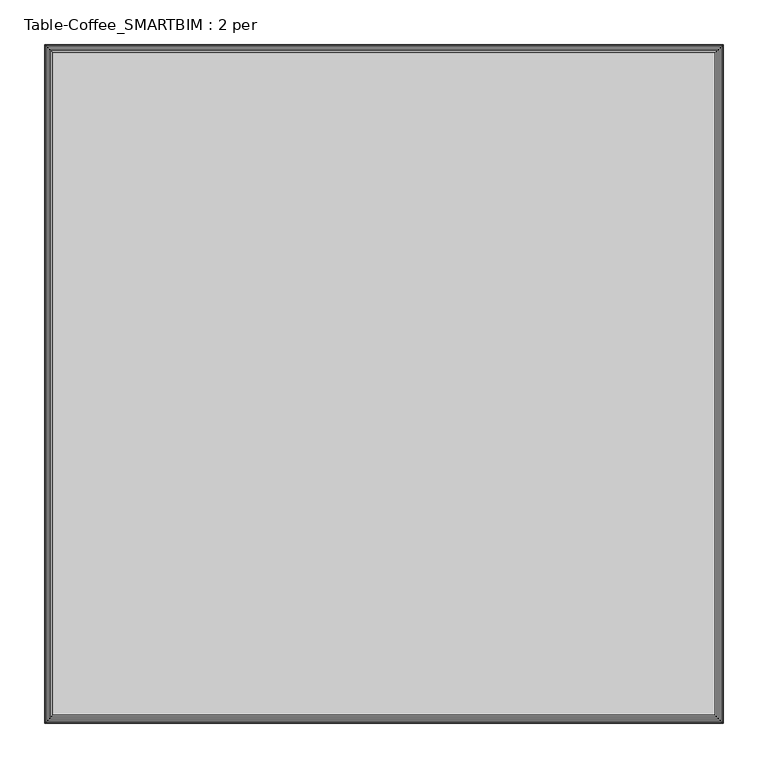
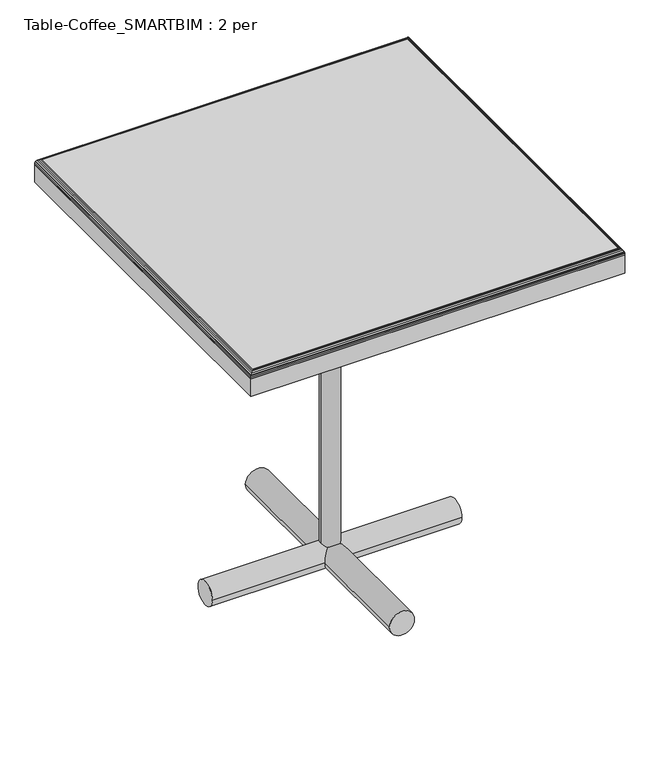
"""IFC4 building model written with IfcOpenShell, lengths in millimetres: furniture geometry, Table-Coffee_SMARTBIM : 2 per."""

from ifc_helpers import new_model, si_unit, point, frame, frame_2d, origin, origin_2d, place, context, project, spatial, polyline, circle_curve, ellipse_curve, trimmed, segment, composite_curve, outline, extrude, source, transform, mapped, element, save
from ifc_brep_helpers import plane_surface, cylinder_surface, advanced_brep


def table_coffee_smartbim_2_per_484a3bd6(model_context):
    return source(origin(), model_context, "Body", "SolidModel", [
        extrude(outline(composite_curve([segment(trimmed(circle_curve(frame_2d((0.0, 25.4)), 25.4), [point((-25.4, 25.4))], [point((25.4, 25.4))], False, "CARTESIAN"), True, "CONTINUOUS"), segment(trimmed(circle_curve(frame_2d((0.0, 25.4)), 25.4), [point((25.4, 25.4))], [point((-25.4, 25.4))], False, "CARTESIAN"), True, "CONTINUOUS")], self_intersect=False)), frame((-254.0, 0.0, 0.0), z_axis=(1.0, 0.0, 0.0), x_axis=(0.0, 1.0, 0.0)), (0.0, 0.0, 1.0), 508.0),
        extrude(outline(composite_curve([segment(trimmed(circle_curve(frame_2d((25.4, 0.0)), 25.4), [point((25.4, -25.4))], [point((25.4, 25.4))], False, "CARTESIAN"), True, "CONTINUOUS"), segment(trimmed(circle_curve(frame_2d((25.4, 0.0)), 25.4), [point((25.4, 25.4))], [point((25.4, -25.4))], False, "CARTESIAN"), True, "CONTINUOUS")], self_intersect=False)), frame((0.0, -254.0, 0.0), z_axis=(0.0, 1.0, 0.0), x_axis=(0.0, 0.0, 1.0)), (0.0, 0.0, 1.0), 508.0),
        extrude(outline(polyline([(381.0, -381.0), (-381.0, -381.0), (-381.0, 381.0), (381.0, 381.0), (381.0, -381.0)])), frame((0.0, 0.0, 723.9), z_axis=(0.0, 0.0, 1.0), x_axis=(1.0, 0.0, 0.0)), (0.0, 0.0, 1.0), 38.1),
        advanced_brep(
        [(-371.5998654, 371.5998654, 774.7), (-371.5998654, -371.5998654, 774.7), (371.5998654, -371.5998654, 774.7), (371.5998654, 371.5998654, 774.7), (381.0, -381.0, 762.0), (-381.0, -381.0, 762.0), (-381.0, 381.0, 762.0), (381.0, 381.0, 762.0), (381.0, -381.0, 765.2998654), (-381.0, -381.0, 765.2998654), (-381.0, 381.0, 765.2998654), (381.0, 381.0, 765.2998654), (-380.6372483, -380.6372483, 767.8860287), (-380.6372483, 380.6372483, 767.8860287), (-373.7616212, -373.7616212, 774.4480533), (-373.7616212, 373.7616212, 774.4480533), (-375.7639185, 375.7639185, 773.7273912), (-375.7639185, -375.7639185, 773.7273912), (-377.8885738, 377.8885738, 772.2866155), (-377.8885738, -377.8885738, 772.2866155), (-379.9102962, 379.9102962, 769.692959), (-379.9102962, -379.9102962, 769.692959), (380.6372483, 380.6372483, 767.8860287), (373.7616212, 373.7616212, 774.4480533), (375.7639185, 375.7639185, 773.7273912), (377.8885738, 377.8885738, 772.2866155), (379.9102962, 379.9102962, 769.692959), (380.6372483, -380.6372483, 767.8860287), (373.7616212, -373.7616212, 774.4480533), (375.7639185, -375.7639185, 773.7273912), (377.8885738, -377.8885738, 772.2866155), (379.9102962, -379.9102962, 769.692959)],
        [
            (0, 1),
            (1, 2),
            (2, 3),
            (3, 0),
            (4, 5),
            (5, 6),
            (6, 7),
            (7, 4),
            (4, 8),
            (8, 9),
            (9, 5),
            (9, 10),
            (10, 6),
            (10, 11),
            (11, 7),
            (11, 8),
            (9, 12, ellipse_curve(frame((-371.5998654, -371.5998654, 765.2998654), z_axis=(-0.7071067811865475, 0.7071067811865475, 0.0), x_axis=(0.7071067811865474, 0.7071067811865476, 0.0)), 13.2937978, 9.4001346)),
            (12, 13),
            (13, 10, ellipse_curve(frame((-371.5998654, 371.5998654, 765.2998654), z_axis=(-0.7071067811865475, -0.7071067811865475, 0.0), x_axis=(-0.7071067811865474, 0.7071067811865476, 0.0)), 13.2937978, 9.4001346)),
            (14, 1, ellipse_curve(frame((-371.5998654, -371.5998654, 765.2998654), z_axis=(-0.7071067811865475, 0.7071067811865475, 0.0), x_axis=(0.7071067811865474, 0.7071067811865476, 0.0)), 13.2937978, 9.4001346)),
            (0, 15, ellipse_curve(frame((-371.5998654, 371.5998654, 765.2998654), z_axis=(-0.7071067811865475, -0.7071067811865475, 0.0), x_axis=(-0.7071067811865474, 0.7071067811865476, 0.0)), 13.2937978, 9.4001346)),
            (15, 14),
            (15, 16, ellipse_curve(frame((-371.5998654, 371.5998654, 765.2998654), z_axis=(-0.7071067811865475, -0.7071067811865475, 0.0), x_axis=(-0.7071067811865474, 0.7071067811865476, 0.0)), 13.2937978, 9.4001346)),
            (16, 17),
            (17, 14, ellipse_curve(frame((-371.5998654, -371.5998654, 765.2998654), z_axis=(-0.7071067811865475, 0.7071067811865475, 0.0), x_axis=(0.7071067811865474, 0.7071067811865476, 0.0)), 13.2937978, 9.4001346)),
            (16, 18, ellipse_curve(frame((-371.5998654, 371.5998654, 765.2998654), z_axis=(-0.7071067811865475, -0.7071067811865475, 0.0), x_axis=(-0.7071067811865474, 0.7071067811865476, 0.0)), 13.2937978, 9.4001346)),
            (18, 19),
            (19, 17, ellipse_curve(frame((-371.5998654, -371.5998654, 765.2998654), z_axis=(-0.7071067811865475, 0.7071067811865475, 0.0), x_axis=(0.7071067811865474, 0.7071067811865476, 0.0)), 13.2937978, 9.4001346)),
            (18, 20, ellipse_curve(frame((-371.5998654, 371.5998654, 765.2998654), z_axis=(-0.7071067811865475, -0.7071067811865475, 0.0), x_axis=(-0.7071067811865474, 0.7071067811865476, 0.0)), 13.2937978, 9.4001346)),
            (20, 21),
            (21, 19, ellipse_curve(frame((-371.5998654, -371.5998654, 765.2998654), z_axis=(-0.7071067811865475, 0.7071067811865475, 0.0), x_axis=(0.7071067811865474, 0.7071067811865476, 0.0)), 13.2937978, 9.4001346)),
            (12, 21, ellipse_curve(frame((-371.5998654, -371.5998654, 765.2998654), z_axis=(-0.7071067811865475, 0.7071067811865475, 0.0), x_axis=(0.7071067811865474, 0.7071067811865476, 0.0)), 13.2937978, 9.4001346)),
            (20, 13, ellipse_curve(frame((-371.5998654, 371.5998654, 765.2998654), z_axis=(-0.7071067811865475, -0.7071067811865475, 0.0), x_axis=(-0.7071067811865474, 0.7071067811865476, 0.0)), 13.2937978, 9.4001346)),
            (13, 22),
            (22, 11, ellipse_curve(frame((371.5998654, 371.5998654, 765.2998654), z_axis=(-0.7071067811865475, 0.7071067811865475, 0.0), x_axis=(0.7071067811865476, 0.7071067811865474, 0.0)), 13.2937978, 9.4001346)),
            (3, 23, ellipse_curve(frame((371.5998654, 371.5998654, 765.2998654), z_axis=(-0.7071067811865475, 0.7071067811865475, 0.0), x_axis=(0.7071067811865476, 0.7071067811865474, 0.0)), 13.2937978, 9.4001346)),
            (23, 15),
            (23, 24, ellipse_curve(frame((371.5998654, 371.5998654, 765.2998654), z_axis=(-0.7071067811865475, 0.7071067811865475, 0.0), x_axis=(0.7071067811865476, 0.7071067811865474, 0.0)), 13.2937978, 9.4001346)),
            (24, 16),
            (24, 25, ellipse_curve(frame((371.5998654, 371.5998654, 765.2998654), z_axis=(-0.7071067811865475, 0.7071067811865475, 0.0), x_axis=(0.7071067811865476, 0.7071067811865474, 0.0)), 13.2937978, 9.4001346)),
            (25, 18),
            (25, 26, ellipse_curve(frame((371.5998654, 371.5998654, 765.2998654), z_axis=(-0.7071067811865475, 0.7071067811865475, 0.0), x_axis=(0.7071067811865476, 0.7071067811865474, 0.0)), 13.2937978, 9.4001346)),
            (26, 20),
            (26, 22, ellipse_curve(frame((371.5998654, 371.5998654, 765.2998654), z_axis=(-0.7071067811865475, 0.7071067811865475, 0.0), x_axis=(0.7071067811865476, 0.7071067811865474, 0.0)), 13.2937978, 9.4001346)),
            (22, 27),
            (27, 8, ellipse_curve(frame((371.5998654, -371.5998654, 765.2998654), z_axis=(0.7071067811865475, 0.7071067811865475, 0.0), x_axis=(0.7071067811865474, -0.7071067811865476, 0.0)), 13.2937978, 9.4001346)),
            (2, 28, ellipse_curve(frame((371.5998654, -371.5998654, 765.2998654), z_axis=(0.7071067811865475, 0.7071067811865475, 0.0), x_axis=(0.7071067811865474, -0.7071067811865476, 0.0)), 13.2937978, 9.4001346)),
            (28, 23),
            (28, 29, ellipse_curve(frame((371.5998654, -371.5998654, 765.2998654), z_axis=(0.7071067811865475, 0.7071067811865475, 0.0), x_axis=(0.7071067811865474, -0.7071067811865476, 0.0)), 13.2937978, 9.4001346)),
            (29, 24),
            (29, 30, ellipse_curve(frame((371.5998654, -371.5998654, 765.2998654), z_axis=(0.7071067811865475, 0.7071067811865475, 0.0), x_axis=(0.7071067811865474, -0.7071067811865476, 0.0)), 13.2937978, 9.4001346)),
            (30, 25),
            (30, 31, ellipse_curve(frame((371.5998654, -371.5998654, 765.2998654), z_axis=(0.7071067811865475, 0.7071067811865475, 0.0), x_axis=(0.7071067811865474, -0.7071067811865476, 0.0)), 13.2937978, 9.4001346)),
            (31, 26),
            (31, 27, ellipse_curve(frame((371.5998654, -371.5998654, 765.2998654), z_axis=(0.7071067811865475, 0.7071067811865475, 0.0), x_axis=(0.7071067811865474, -0.7071067811865476, 0.0)), 13.2937978, 9.4001346)),
            (27, 12),
            (14, 28),
            (17, 29),
            (19, 30),
            (21, 31),
        ],
        [
            plane_surface(frame((-381.0, -381.0, 774.7), z_axis=(0.0, 0.0, 1.0), x_axis=(-1.0, 0.0, 0.0))),
            plane_surface(frame((-381.0, -381.0, 762.0), z_axis=(0.0, 0.0, -1.0), x_axis=(1.0, 0.0, 0.0))),
            plane_surface(frame((381.0, -381.0, 774.7), z_axis=(0.0, -1.0, 0.0), x_axis=(0.0, 0.0, -1.0))),
            plane_surface(frame((-381.0, -381.0, 774.7), z_axis=(-1.0, 0.0, 0.0), x_axis=(0.0, 0.0, -1.0))),
            plane_surface(frame((-381.0, 381.0, 774.7), z_axis=(0.0, 1.0, 0.0), x_axis=(0.0, 0.0, -1.0))),
            plane_surface(frame((381.0, 381.0, 774.7), z_axis=(1.0, 0.0, 0.0), x_axis=(0.0, 0.0, -1.0))),
            cylinder_surface(frame((-371.5998654, -381.0, 765.2998654), z_axis=(0.0, 1.0, 0.0), x_axis=(1.0, 0.0, 0.0)), 9.4001346),
            cylinder_surface(frame((-381.0, 371.5998654, 765.2998654), z_axis=(1.0, 0.0, 0.0), x_axis=(0.0, -1.0, 0.0)), 9.4001346),
            cylinder_surface(frame((371.5998654, 381.0, 765.2998654), z_axis=(0.0, -1.0, 0.0), x_axis=(-1.0, 0.0, 0.0)), 9.4001346),
            cylinder_surface(frame((381.0, -371.5998654, 765.2998654), z_axis=(-1.0, 0.0, 0.0), x_axis=(0.0, 1.0, 0.0)), 9.4001346),
        ],
        [
            (0, [[1, 2, 3, 4]]),
            (1, [[5, 6, 7, 8]]),
            (2, [[9, 10, 11, -5]]),
            (3, [[-11, 12, 13, -6]]),
            (4, [[-13, 14, 15, -7]]),
            (5, [[-15, 16, -9, -8]]),
            (6, [[-12, 17, 18, 19]]),
            (6, [[20, -1, 21, 22]]),
            (6, [[23, 24, 25, -22]]),
            (6, [[26, 27, 28, -24]]),
            (6, [[29, 30, 31, -27]]),
            (6, [[32, -30, 33, -18]]),
            (7, [[34, 35, -14, -19]]),
            (7, [[-4, 36, 37, -21]]),
            (7, [[-37, 38, 39, -23]]),
            (7, [[-39, 40, 41, -26]]),
            (7, [[-41, 42, 43, -29]]),
            (7, [[-43, 44, -34, -33]]),
            (8, [[45, 46, -16, -35]]),
            (8, [[-3, 47, 48, -36]]),
            (8, [[-48, 49, 50, -38]]),
            (8, [[-50, 51, 52, -40]]),
            (8, [[-52, 53, 54, -42]]),
            (8, [[-54, 55, -45, -44]]),
            (9, [[-10, -46, 56, -17]]),
            (9, [[57, -47, -2, -20]]),
            (9, [[58, -49, -57, -25]]),
            (9, [[59, -51, -58, -28]]),
            (9, [[60, -53, -59, -31]]),
            (9, [[-56, -55, -60, -32]]),
        ],
    ),
        extrude(outline(polyline([(76.2, -76.2), (-76.2, -76.2), (-76.2, 76.2), (76.2, 76.2), (76.2, -76.2)])), frame((0.0, 0.0, 755.65), z_axis=(0.0, 0.0, 1.0), x_axis=(1.0, 0.0, 0.0)), (0.0, 0.0, 1.0), 6.35),
        extrude(outline(composite_curve([segment(trimmed(circle_curve(origin_2d(), 19.05), [point((-19.05, 0.0))], [point((19.05, 0.0))], False, "CARTESIAN"), True, "CONTINUOUS"), segment(trimmed(circle_curve(origin_2d(), 19.05), [point((19.05, 0.0))], [point((-19.05, 0.0))], False, "CARTESIAN"), True, "CONTINUOUS")], self_intersect=False)), frame((0.0, 0.0, 24.2070278), z_axis=(0.0, 0.0, 1.0), x_axis=(1.0, 0.0, 0.0)), (0.0, 0.0, 1.0), 731.4429722),
    ])


if __name__ == "__main__":
    model = new_model("IFC4")
    model_context = context("Model", 3, world=origin())
    ifc_project = project(units=[si_unit("LENGTHUNIT", "METRE", prefix="MILLI")], contexts=[model_context])
    site = spatial("IfcSite", under=ifc_project)
    building = spatial("IfcBuilding", under=site)
    placement = place(None, origin())
    table_coffee_smartbim_2_per_shape = table_coffee_smartbim_2_per_484a3bd6(model_context)
    element("IfcFurniture", 1, ObjectType="Table-Coffee_SMARTBIM : 2 per", at=placement, inside=building, context=model_context, shape_type="MappedRepresentation", body=[
        mapped(table_coffee_smartbim_2_per_shape, transform((0.0, 0.0, 0.0), x_axis=(1.0, 0.0, 0.0), y_axis=(0.0, 1.0, 0.0), z_axis=(0.0, 0.0, 1.0))),
    ])
    save(model, "model.ifc")

# Revit data of these elements
# Type "Table-Coffee_SMARTBIM : 2 per"
#   Subcategory = "Table\r\n"
#   SmartBIM Object Created By = "SMARTBIM, LLC"
#   Manufacturer = "SMARTBIM"
#   Assembly Code = "E2020200"
#   95 CSI = "12500"
#   04 CSI = "12 50 00"
#   table cloth = 0' - 1 1/2"
#   Width = 2' - 6"
#   SmartBIM Object Version = 3
#   Height = 2' - 6"
#   Depth = 2' - 6"
#   Default Elevation = 4' - 0"
#   white cloth_parameter = WOOD-OAKFIRE
#   Table Unit = MET
#   Glide = none
#   Glass = none
# Element 1 (IfcFurniture, "Table-Coffee_SMARTBIM : 2 per")
#   Materials on its faces: "WOOD-OAKFIRE", "MET"
# Materials
#   "WOOD-OAKFIRE": class "Wood", colour RGB 198 202 183, transparency 0, Description = "Generic wood", Cost = 0
#   "MET": class "Metal", colour RGB 189 187 185, transparency 0
